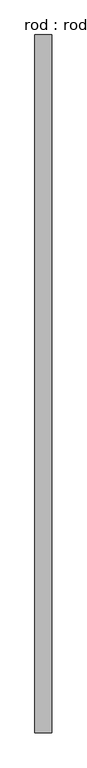
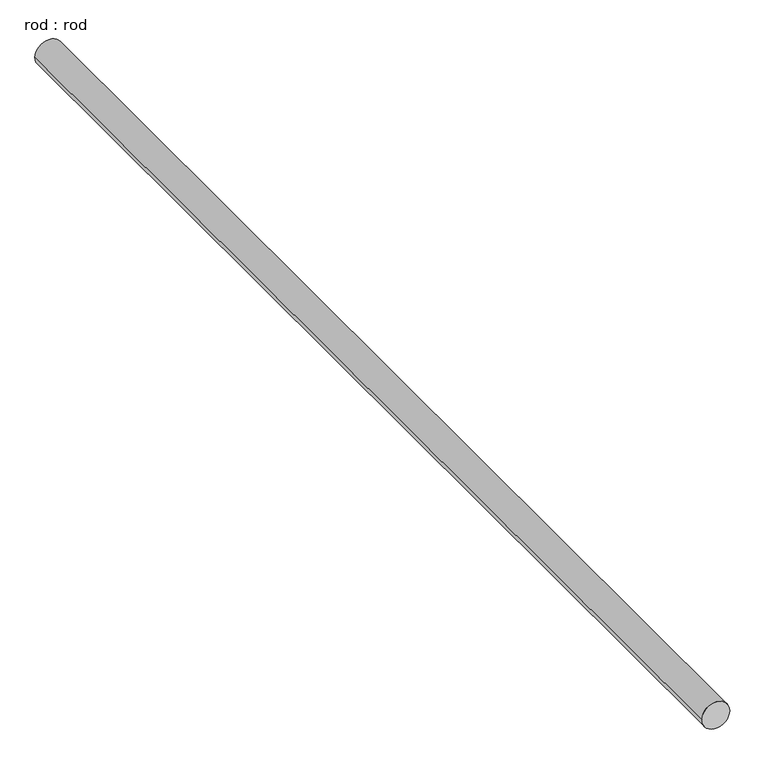
"""IFC4 building model written with IfcOpenShell, lengths in millimetres: proxy geometry, rod : rod."""

from ifc_helpers import new_model, si_unit, point, frame, frame_2d, origin, place, context, project, spatial, circle_curve, trimmed, segment, composite_curve, outline, extrude, source, transform, mapped, element, save


def rod_rod_67964f64(model_context):
    return source(origin(), model_context, "Body", "SweptSolid", [
        extrude(outline(composite_curve([segment(trimmed(circle_curve(frame_2d((0.0108462, 0.0)), 200.0), [point((0.0108462, 200.0))], [point((0.0108462, -200.0))], False, "CARTESIAN"), True, "CONTINUOUS"), segment(trimmed(circle_curve(frame_2d((0.0108462, 0.0)), 200.0), [point((0.0108462, -200.0))], [point((0.0108462, 200.0))], False, "CARTESIAN"), True, "CONTINUOUS")], self_intersect=False)), frame((0.0, -4157.2713847, 0.0), z_axis=(0.0, 1.0, 0.0), x_axis=(0.0, 0.0, 1.0)), (0.0, 0.0, 1.0), 16500.0),
    ])


if __name__ == "__main__":
    model = new_model("IFC4")
    model_context = context("Model", 3, world=origin())
    ifc_project = project(units=[si_unit("LENGTHUNIT", "METRE", prefix="MILLI")], contexts=[model_context])
    site = spatial("IfcSite", under=ifc_project)
    building = spatial("IfcBuilding", under=site)
    placement = place(None, origin())
    rod_rod_shape = rod_rod_67964f64(model_context)
    element("IfcBuildingElementProxy", 1, Name="rod : rod", ObjectType="rod : rod", at=placement, inside=building, context=model_context, shape_type="MappedRepresentation", body=[
        mapped(rod_rod_shape, transform((0.0, 0.0, 0.0), x_axis=(1.0, 0.0, 0.0), y_axis=(0.0, 1.0, 0.0), z_axis=(0.0, 0.0, 1.0))),
    ])
    save(model, "model.ifc")

# Revit data of these elements
# Type "rod : rod"
#   Default Elevation = 0
